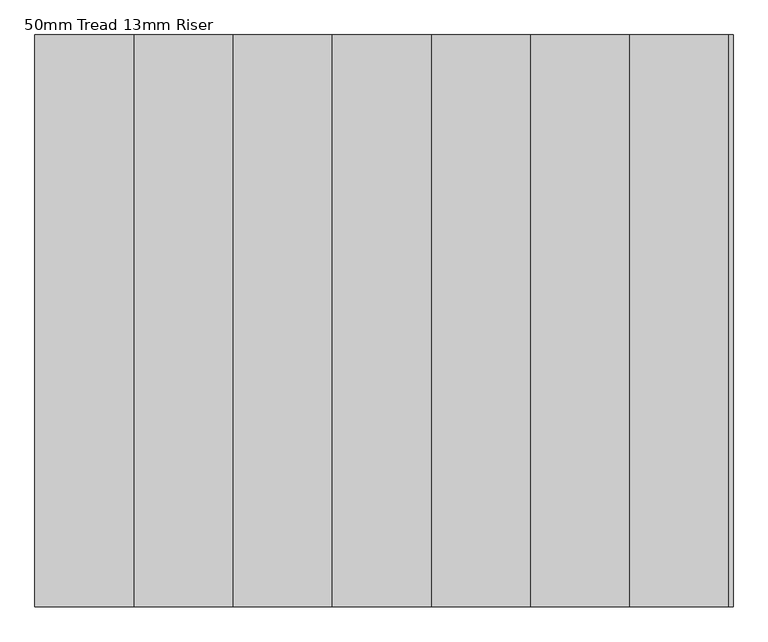
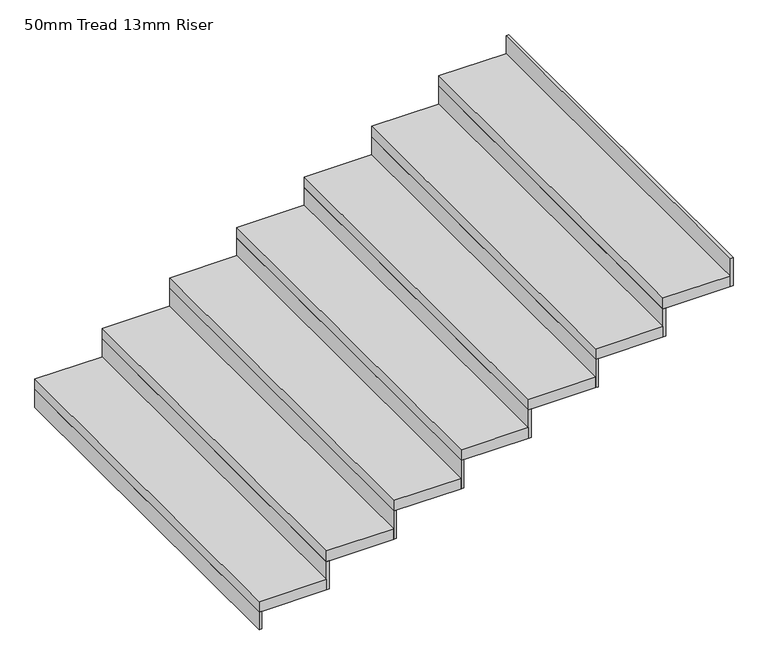
"""IFC4 building model written with IfcOpenShell, lengths in millimetres: stair flight geometry, 50mm Tread 13mm Riser."""

from ifc_helpers import new_model, si_unit, frame, origin, place, context, project, spatial, polyline, outline, extrude, source, transform, mapped, element, save


def stair_flight_50mm_tread_13mm_riser_cadf6dc6(model_context):
    return source(origin(), model_context, "Body", "SweptSolid", [
        extrude(outline(polyline([(-15531.918089, 15530.6768963), (-15544.418089, 15530.6768963), (-15544.418089, 17260.6768963), (-15531.918089, 17260.6768963), (-15531.918089, 15530.6768963)])), frame((0.0, 0.0, -1066.6666667), z_axis=(0.0, 0.0, 1.0), x_axis=(1.0, 0.0, 0.0)), (0.0, 0.0, 1.0), 83.3333333),
        extrude(outline(polyline([(-15244.418089, 17260.6768963), (-15244.418089, 15530.6768963), (-15544.418089, 15530.6768963), (-15544.418089, 17260.6768963), (-15244.418089, 17260.6768963)])), frame((0.0, 0.0, -983.3333333), z_axis=(0.0, 0.0, 1.0), x_axis=(1.0, 0.0, 0.0)), (0.0, 0.0, 1.0), 50.0),
        extrude(outline(polyline([(-15231.918089, 15530.6768963), (-15244.418089, 15530.6768963), (-15244.418089, 17260.6768963), (-15231.918089, 17260.6768963), (-15231.918089, 15530.6768963)])), frame((0.0, 0.0, -983.3333333), z_axis=(0.0, 0.0, 1.0), x_axis=(1.0, 0.0, 0.0)), (0.0, 0.0, 1.0), 133.3333333),
        extrude(outline(polyline([(-14944.418089, 17260.6768963), (-14944.418089, 15530.6768963), (-15244.418089, 15530.6768963), (-15244.418089, 17260.6768963), (-14944.418089, 17260.6768963)])), frame((0.0, 0.0, -850.0), z_axis=(0.0, 0.0, 1.0), x_axis=(1.0, 0.0, 0.0)), (0.0, 0.0, 1.0), 50.0),
        extrude(outline(polyline([(-14931.918089, 15530.6768963), (-14944.418089, 15530.6768963), (-14944.418089, 17260.6768963), (-14931.918089, 17260.6768963), (-14931.918089, 15530.6768963)])), frame((0.0, 0.0, -850.0), z_axis=(0.0, 0.0, 1.0), x_axis=(1.0, 0.0, 0.0)), (0.0, 0.0, 1.0), 133.3333333),
        extrude(outline(polyline([(-14644.418089, 17260.6768963), (-14644.418089, 15530.6768963), (-14944.418089, 15530.6768963), (-14944.418089, 17260.6768963), (-14644.418089, 17260.6768963)])), frame((0.0, 0.0, -716.6666667), z_axis=(0.0, 0.0, 1.0), x_axis=(1.0, 0.0, 0.0)), (0.0, 0.0, 1.0), 50.0),
        extrude(outline(polyline([(-14631.918089, 15530.6768963), (-14644.418089, 15530.6768963), (-14644.418089, 17260.6768963), (-14631.918089, 17260.6768963), (-14631.918089, 15530.6768963)])), frame((0.0, 0.0, -716.6666667), z_axis=(0.0, 0.0, 1.0), x_axis=(1.0, 0.0, 0.0)), (0.0, 0.0, 1.0), 133.3333333),
        extrude(outline(polyline([(-14344.418089, 17260.6768963), (-14344.418089, 15530.6768963), (-14644.418089, 15530.6768963), (-14644.418089, 17260.6768963), (-14344.418089, 17260.6768963)])), frame((0.0, 0.0, -583.3333333), z_axis=(0.0, 0.0, 1.0), x_axis=(1.0, 0.0, 0.0)), (0.0, 0.0, 1.0), 50.0),
        extrude(outline(polyline([(-14331.918089, 15530.6768963), (-14344.418089, 15530.6768963), (-14344.418089, 17260.6768963), (-14331.918089, 17260.6768963), (-14331.918089, 15530.6768963)])), frame((0.0, 0.0, -583.3333333), z_axis=(0.0, 0.0, 1.0), x_axis=(1.0, 0.0, 0.0)), (0.0, 0.0, 1.0), 133.3333333),
        extrude(outline(polyline([(-14044.418089, 17260.6768963), (-14044.418089, 15530.6768963), (-14344.418089, 15530.6768963), (-14344.418089, 17260.6768963), (-14044.418089, 17260.6768963)])), frame((0.0, 0.0, -450.0), z_axis=(0.0, 0.0, 1.0), x_axis=(1.0, 0.0, 0.0)), (0.0, 0.0, 1.0), 50.0),
        extrude(outline(polyline([(-14031.918089, 15530.6768963), (-14044.418089, 15530.6768963), (-14044.418089, 17260.6768963), (-14031.918089, 17260.6768963), (-14031.918089, 15530.6768963)])), frame((0.0, 0.0, -450.0), z_axis=(0.0, 0.0, 1.0), x_axis=(1.0, 0.0, 0.0)), (0.0, 0.0, 1.0), 133.3333333),
        extrude(outline(polyline([(-13744.418089, 17260.6768963), (-13744.418089, 15530.6768963), (-14044.418089, 15530.6768963), (-14044.418089, 17260.6768963), (-13744.418089, 17260.6768963)])), frame((0.0, 0.0, -316.6666667), z_axis=(0.0, 0.0, 1.0), x_axis=(1.0, 0.0, 0.0)), (0.0, 0.0, 1.0), 50.0),
        extrude(outline(polyline([(-13731.918089, 15530.6768963), (-13744.418089, 15530.6768963), (-13744.418089, 17260.6768963), (-13731.918089, 17260.6768963), (-13731.918089, 15530.6768963)])), frame((0.0, 0.0, -316.6666667), z_axis=(0.0, 0.0, 1.0), x_axis=(1.0, 0.0, 0.0)), (0.0, 0.0, 1.0), 133.3333333),
        extrude(outline(polyline([(-13431.918089, 15530.6768963), (-13444.418089, 15530.6768963), (-13444.418089, 17260.6768963), (-13431.918089, 17260.6768963), (-13431.918089, 15530.6768963)])), frame((0.0, 0.0, -183.3333333), z_axis=(0.0, 0.0, 1.0), x_axis=(1.0, 0.0, 0.0)), (0.0, 0.0, 1.0), 133.3333333),
        extrude(outline(polyline([(-13444.418089, 17260.6768963), (-13444.418089, 15530.6768963), (-13744.418089, 15530.6768963), (-13744.418089, 17260.6768963), (-13444.418089, 17260.6768963)])), frame((0.0, 0.0, -183.3333333), z_axis=(0.0, 0.0, 1.0), x_axis=(1.0, 0.0, 0.0)), (0.0, 0.0, 1.0), 50.0),
    ])


if __name__ == "__main__":
    model = new_model("IFC4")
    model_context = context("Model", 3, world=origin())
    ifc_project = project(units=[si_unit("LENGTHUNIT", "METRE", prefix="MILLI")], contexts=[model_context])
    site = spatial("IfcSite", under=ifc_project)
    building = spatial("IfcBuilding", under=site)
    placement = place(None, origin())
    stair_flight_50mm_tread_13mm_riser_shape = stair_flight_50mm_tread_13mm_riser_cadf6dc6(model_context)
    element("IfcStairFlight", 1, ObjectType="50mm Tread 13mm Riser", at=placement, inside=building, context=model_context, shape_type="MappedRepresentation", body=[
        mapped(stair_flight_50mm_tread_13mm_riser_shape, transform((0.0, 0.0, 0.0), x_axis=(1.0, 0.0, 0.0), y_axis=(0.0, 1.0, 0.0), z_axis=(0.0, 0.0, 1.0))),
    ])
    save(model, "model.ifc")
